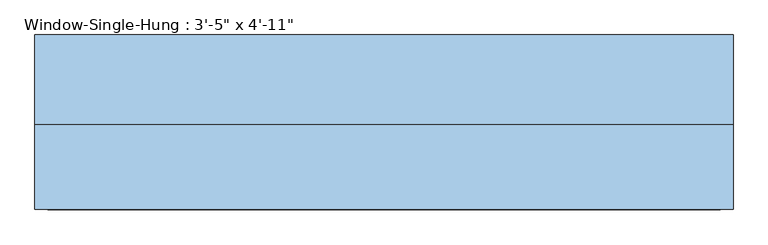
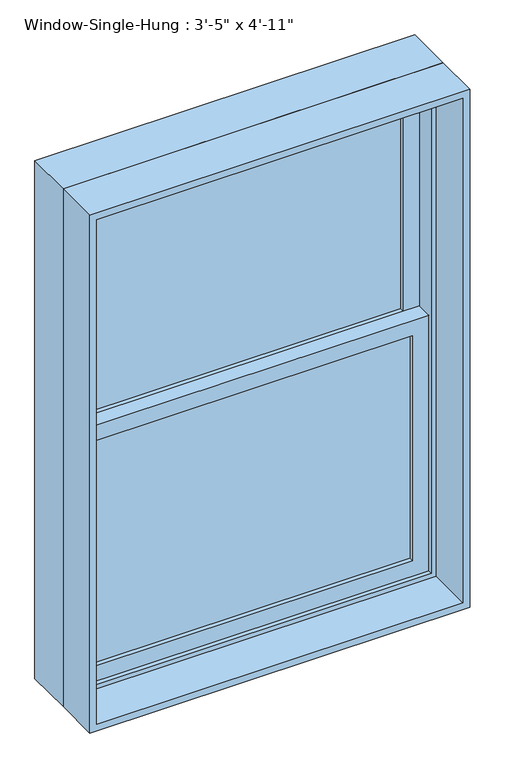
"""IFC4 building model written with IfcOpenShell, lengths in millimetres: window geometry."""

import ifcopenshell
import ifcopenshell.guid

model = None  # the IFC model being written
_history = None  # IfcOwnerHistory: only IFC2X3 demands one
_inside = {}  # id of a spatial element -> (the spatial element, [elements in it])
_under = {}  # id of a project, library or spatial element -> (it, [spatial elements below it])
_declared = {}  # id of a project -> (the project, [libraries it declares])
_typed = {}  # id of a type object -> (the type object, [elements of that type])
_made_of = {}  # id of a material, layer set ... -> (it, [elements and type objects made of it])


def new_model(schema):
    """Start an empty IFC model of exactly this schema.

    Asked for "IFC4X3", IfcOpenShell would pick the latest addendum, in which some entities
    have other attributes; the version numbers below select the first issue.
    IFC2X3 requires an IfcOwnerHistory on every rooted entity: one is made here for all.
    """
    global model, _history
    if schema == "IFC4X3":
        model = ifcopenshell.file(schema_version=(4, 3, 0, 0))
    else:
        model = ifcopenshell.file(schema=schema)
    _inside.clear()
    _under.clear()
    _declared.clear()
    _typed.clear()
    _made_of.clear()
    _history = None
    if model.schema == "IFC2X3":
        org = make("IfcOrganization", Name="unknown")
        user = make(
            "IfcPersonAndOrganization",
            ThePerson=make("IfcPerson", FamilyName="unknown"),
            TheOrganization=org,
        )
        app = make(
            "IfcApplication",
            ApplicationDeveloper=org,
            Version="unknown",
            ApplicationFullName="unknown",
            ApplicationIdentifier="unknown",
        )
        _history = make(
            "IfcOwnerHistory",
            OwningUser=user,
            OwningApplication=app,
            ChangeAction="ADDED",
            CreationDate=0,
        )
    return model


def make(cls, **values):
    """One entity of the class cls with the attributes given. An attribute that is None is left unset."""
    return model.create_entity(
        cls, **{name: value for name, value in values.items() if value is not None}
    )


def rooted(cls, **values):
    """An entity with a GlobalId (a new one), such as an element, a storey or a relation."""
    return make(cls, GlobalId=ifcopenshell.guid.new(), OwnerHistory=_history, **values)


def si_unit(unit_type, name, prefix=None):
    """IfcSIUnit, for example si_unit("LENGTHUNIT", "METRE", prefix="MILLI")."""
    return make("IfcSIUnit", UnitType=unit_type, Prefix=prefix, Name=name)


def assignment(units):
    """IfcUnitAssignment: the units of a project."""
    return None if units is None else make("IfcUnitAssignment", Units=units)


def point(xyz):
    """IfcCartesianPoint."""
    return None if xyz is None else make("IfcCartesianPoint", Coordinates=xyz)


def direction(xyz):
    """IfcDirection."""
    return None if xyz is None else make("IfcDirection", DirectionRatios=xyz)


def frame(location, z_axis=None, x_axis=None):
    """IfcAxis2Placement3D, a coordinate frame: its origin and axes. An axis left out is left unset."""
    return make(
        "IfcAxis2Placement3D",
        Location=point(location),
        Axis=direction(z_axis),
        RefDirection=direction(x_axis),
    )


def origin():
    """The frame at (0, 0, 0) with its axes left unset."""
    return frame((0.0, 0.0, 0.0))


def place(relative_to, where):
    """IfcLocalPlacement: puts the frame where relative to a parent placement (None: the world)."""
    return make(
        "IfcLocalPlacement", PlacementRelTo=relative_to, RelativePlacement=where
    )


def context(
    kind, dimensions, precision=None, world=None, true_north=None, identifier=None
):
    """IfcGeometricRepresentationContext, for example the 3D "Model" context."""
    return make(
        "IfcGeometricRepresentationContext",
        ContextIdentifier=identifier,
        ContextType=kind,
        CoordinateSpaceDimension=dimensions,
        Precision=precision,
        WorldCoordinateSystem=world,
        TrueNorth=true_north,
    )


def project(units=None, contexts=None):
    """IfcProject with its units and contexts."""
    return rooted(
        "IfcProject",
        Name="project",
        RepresentationContexts=contexts,
        UnitsInContext=assignment(units),
    )


def spatial(cls, under=None, at=None, **own):
    """A site, building, storey or space (cls), placed at a placement, below another one or the project."""
    s = rooted(cls, ObjectPlacement=at, **own)
    if under is not None:
        _under.setdefault(under.id(), (under, []))[1].append(s)
    return s


def polyline(points):
    """IfcPolyline through the points."""
    return make("IfcPolyline", Points=[point(p) for p in points])


def outline(outer, holes=None, kind="AREA"):
    """IfcArbitraryClosedProfileDef: a profile drawn as a closed curve; with holes, ...WithVoids."""
    if holes is None:
        return make("IfcArbitraryClosedProfileDef", ProfileType=kind, OuterCurve=outer)
    return make(
        "IfcArbitraryProfileDefWithVoids",
        ProfileType=kind,
        OuterCurve=outer,
        InnerCurves=holes,
    )


def extrude(swept, where, along, depth):
    """IfcExtrudedAreaSolid: the profile swept, set in the frame where, extruded along a direction by depth."""
    return make(
        "IfcExtrudedAreaSolid",
        SweptArea=swept,
        Position=where,
        ExtrudedDirection=direction(along),
        Depth=depth,
    )


def shape(context_of_items, identifier, shape_type, items):
    """IfcShapeRepresentation: the items that make up one representation, for example the "Body"."""
    return make(
        "IfcShapeRepresentation",
        ContextOfItems=context_of_items,
        RepresentationIdentifier=identifier,
        RepresentationType=shape_type,
        Items=items,
    )


def source(mapping_origin, context_of_items, identifier, shape_type, items):
    """IfcRepresentationMap: a shape defined once, which mapped items show again and again."""
    return make(
        "IfcRepresentationMap",
        MappingOrigin=mapping_origin,
        MappedRepresentation=shape(context_of_items, identifier, shape_type, items),
    )


def transform(
    local_origin,
    x_axis=None,
    y_axis=None,
    z_axis=None,
    scale=None,
    scale2=None,
    scale3=None,
    uniform=True,
):
    """IfcCartesianTransformationOperator3D, or its non-uniform kind. x_axis, y_axis, z_axis: its Axis1, 2, 3."""
    if uniform:
        return make(
            "IfcCartesianTransformationOperator3D",
            Axis1=direction(x_axis),
            Axis2=direction(y_axis),
            LocalOrigin=point(local_origin),
            Scale=scale,
            Axis3=direction(z_axis),
        )
    return make(
        "IfcCartesianTransformationOperator3DnonUniform",
        Axis1=direction(x_axis),
        Axis2=direction(y_axis),
        LocalOrigin=point(local_origin),
        Scale=scale,
        Axis3=direction(z_axis),
        Scale2=scale2,
        Scale3=scale3,
    )


def mapped(mapping_source, mapping_target):
    """IfcMappedItem: shows the shape of a source again, moved by a transform."""
    return make(
        "IfcMappedItem", MappingSource=mapping_source, MappingTarget=mapping_target
    )


def made_of(thing, what):
    """Note that an element or type object is made of a material, layer set ...; save() writes the relation."""
    if what is not None:
        _made_of.setdefault(what.id(), (what, []))[1].append(thing)
    return thing


def element(
    cls,
    number,
    at=None,
    inside=None,
    cuts=None,
    type_object=None,
    material=None,
    context=None,
    identifier="Body",
    shape_type=None,
    held_by="IfcProductDefinitionShape",
    body=None,
    shapes=None,
    **own,
):
    """One element of the class cls, such as IfcWall. Its Tag is "e" and its number.

    at: its placement. inside: the storey or other place that contains it. cuts: it is an
    opening in that element (IfcRelVoidsElement). A single representation is given by context,
    identifier, shape_type and body (its items); several are given by shapes. held_by: the class
    of the entity that holds the representations. save() writes the other relations.
    """
    e = rooted(cls, Tag="e%d" % number, ObjectPlacement=at, **own)
    if body is not None:
        shapes = [shape(context, identifier, shape_type, body)]
    if shapes is not None:
        e.Representation = make(held_by, Representations=shapes)
    if inside is not None:
        _inside.setdefault(inside.id(), (inside, []))[1].append(e)
    if cuts is not None:
        rooted(
            "IfcRelVoidsElement", RelatingBuildingElement=cuts, RelatedOpeningElement=e
        )
    if type_object is not None:
        _typed.setdefault(type_object.id(), (type_object, []))[1].append(e)
    return made_of(e, material)


def aggregate(whole, parts):
    """IfcRelAggregates: a whole, such as a stair, and the parts it consists of."""
    return rooted("IfcRelAggregates", RelatingObject=whole, RelatedObjects=parts)


def save(model, path):
    """Write the relations noted so far, then the file.

    IfcRelAggregates (storeys below a building ...), IfcRelContainedInSpatialStructure (elements
    in a storey), IfcRelDefinesByType, IfcRelAssociatesMaterial and IfcRelDeclares: one each for
    every whole, place, type object, material and project.
    """
    for whole, parts in _under.values():
        aggregate(whole, parts)
    for where, things in _inside.values():
        rooted(
            "IfcRelContainedInSpatialStructure",
            RelatedElements=things,
            RelatingStructure=where,
        )
    for kind, things in _typed.values():
        rooted("IfcRelDefinesByType", RelatedObjects=things, RelatingType=kind)
    for what, things in _made_of.values():
        rooted("IfcRelAssociatesMaterial", RelatedObjects=things, RelatingMaterial=what)
    for by, libraries in _declared.values():
        rooted("IfcRelDeclares", RelatingContext=by, RelatedDefinitions=libraries)
    model.write(path)


def window_84eda538(model_context):
    return source(origin(), model_context, "Body", "SweptSolid", [
        extrude(outline(polyline([(444.5, 50.8), (444.5, 44.45), (-444.5, 44.45), (-444.5, 50.8), (444.5, 50.8)])), frame((0.0, 0.0, 990.6), z_axis=(0.0, 0.0, 1.0), x_axis=(1.0, 0.0, 0.0)), (0.0, 0.0, 1.0), 650.875),
        extrude(outline(polyline([(-444.5, 38.1), (444.5, 38.1), (444.5, 31.75), (-444.5, 31.75), (-444.5, 38.1)])), frame((0.0, 0.0, 990.6), z_axis=(0.0, 0.0, 1.0), x_axis=(1.0, 0.0, 0.0)), (0.0, 0.0, 1.0), 650.875),
        extrude(outline(polyline([(444.5, 95.25), (444.5, 88.9), (-444.5, 88.9), (-444.5, 95.25), (444.5, 95.25)])), frame((0.0, 0.0, 1685.925), z_axis=(0.0, 0.0, 1.0), x_axis=(1.0, 0.0, 0.0)), (0.0, 0.0, 1.0), 650.875),
        extrude(outline(polyline([(-444.5, 82.55), (444.5, 82.55), (444.5, 76.2), (-444.5, 76.2), (-444.5, 82.55)])), frame((0.0, 0.0, 1685.925), z_axis=(0.0, 0.0, 1.0), x_axis=(1.0, 0.0, 0.0)), (0.0, 0.0, 1.0), 650.875),
        extrude(outline(polyline([(1685.925, -488.95), (946.15, -488.95), (946.15, 488.95), (1685.925, 488.95), (1685.925, -488.95)]), holes=[polyline([(1641.475, 444.5), (990.6, 444.5), (990.6, -444.5), (1641.475, -444.5), (1641.475, 444.5)])]), frame((0.0, 19.05, 0.0), z_axis=(0.0, 1.0, 0.0), x_axis=(0.0, 0.0, 1.0)), (0.0, 0.0, 1.0), 44.45),
        extrude(outline(polyline([(2381.25, -488.95), (1641.475, -488.95), (1641.475, 488.95), (2381.25, 488.95), (2381.25, -488.95)]), holes=[polyline([(2336.8, 444.5), (1685.925, 444.5), (1685.925, -444.5), (2336.8, -444.5), (2336.8, 444.5)])]), frame((0.0, 63.5, 0.0), z_axis=(0.0, 1.0, 0.0), x_axis=(0.0, 0.0, 1.0)), (0.0, 0.0, 1.0), 44.45),
        extrude(outline(polyline([(2413.0, -520.7), (914.4, -520.7), (914.4, 520.7), (2413.0, 520.7), (2413.0, -520.7)]), holes=[polyline([(2381.25, 488.95), (946.15, 488.95), (946.15, -488.95), (2381.25, -488.95), (2381.25, 488.95)])]), frame((0.0, 6.35, 0.0), z_axis=(0.0, 1.0, 0.0), x_axis=(0.0, 0.0, 1.0)), (0.0, 0.0, 1.0), 133.35),
        extrude(outline(polyline([(2413.0, 520.7), (2413.0, -520.7), (914.4, -520.7), (914.4, 520.7), (2413.0, 520.7)]), holes=[polyline([(2393.95, 501.65), (933.45, 501.65), (933.45, -501.65), (2393.95, -501.65), (2393.95, 501.65)])]), frame((0.0, -120.65, 0.0), z_axis=(0.0, 1.0, 0.0), x_axis=(0.0, 0.0, 1.0)), (0.0, 0.0, 1.0), 127.0),
    ])


if __name__ == "__main__":
    model = new_model("IFC4")
    model_context = context("Model", 3, world=origin())
    ifc_project = project(units=[si_unit("LENGTHUNIT", "METRE", prefix="MILLI")], contexts=[model_context])
    site = spatial("IfcSite", under=ifc_project)
    building = spatial("IfcBuilding", under=site)
    placement = place(None, origin())
    window_shape = window_84eda538(model_context)
    element("IfcWindow", 1, ObjectType="Window-Single-Hung : 3'-5\" x 4'-11\"", at=placement, inside=building, context=model_context, shape_type="MappedRepresentation", body=[
        mapped(window_shape, transform((0.0, 0.0, 0.0), x_axis=(1.0, 0.0, 0.0), y_axis=(0.0, 1.0, 0.0), z_axis=(0.0, 0.0, 1.0))),
    ])
    save(model, "model.ifc")

# Revit data of these elements
# Type "Window-Single-Hung : 3'-5\" x 4'-11\""
#   Type Mark = "21"
#   Fire Rating = "0.5h"
#   Construction Type Id = "DG-DR"
#   Assembly Code = "B2020100"
#   Analytic Construction = "Double glazing - domestic"
#   Wall Thickness [instance default] = 0' - 6"
#   Window Inset [instance default] = 0' - 0"
#   Visual Light Transmittance = 0.81
#   Thermal Resistance (R) = 0.319569 (m²·K)/W
#   Solar Heat Gain Coefficient = 0.76
#   Muntin Width = 2' - 11"
#   Muntin Height = 2' - 1 5/8"
#   Interior Wall Closure [instance default] = 0' - 1 1/2"
#   Rough Width = 3' - 5 1/2"
#   Rough Height = 4' - 11 1/2"
#   Frame Extension [instance default] = 0' - 1 1/4"
#   Exterior Wall Closure [instance default] = 0' - 0 1/2"
#   Extension Jamb [instance default] = 0' - 1 1/2"
#   Heat Transfer Coefficient (U) = 3.12929 W/(m²·K)
#   Height = 4' - 11"
#   Width = 3' - 5"
#   Top Muntin Visibility = no
#   Indicator Visibility = no
#   Extension Jamb Visibility [instance default] = yes
#   Interior Trim Visibility [instance default] = yes
#   Exterior Trim Visibility [instance default] = yes
#   Bottom Muntin Visibility = no
#   Muntin Pattern = Muntin Pattern_2x2 : Muntin Pattern_2x2
#   Interior Trim Material = Wood - Stained
#   Interior Trim = Trim-Window-Interior-Flat : Picture Frame
#   Exterior Trim Material = Clad - White
#   Exterior Trim = Trim-Window-Exterior-Flat : with Sill
#   Glass Panel Material = Glass
#   Exterior Frame Material = Clad - White
#   Interior Frame Material = Wood - Stained
#   Wall Closure = (empty or 0)
# Element 1 (IfcWindow, "Window-Single-Hung : 3'-5\" x 4'-11\"")
#   Wall Thickness = 0' - 9 1/2"
#   Extension Jamb = 0' - 5"
#   Materials on its faces: "Wood - Stained", "Glass", "Clad - White"
# Materials
#   "Wood - Stained": class "Wood", colour RGB 224 178 126, transparency 0, Cost = 0
#   "Clad - White": class "Wood", colour RGB 242 242 238, transparency 0, Cost = 0
#   "Glass": class "Glass", colour RGB 218 227 224, transparency 0.85, Description = "Soda Lime Glass", Cost = 0
